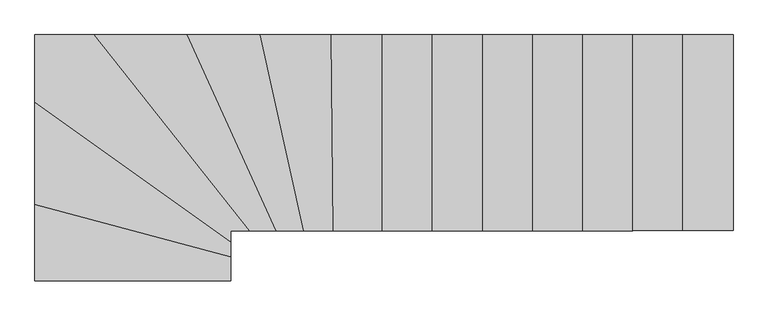
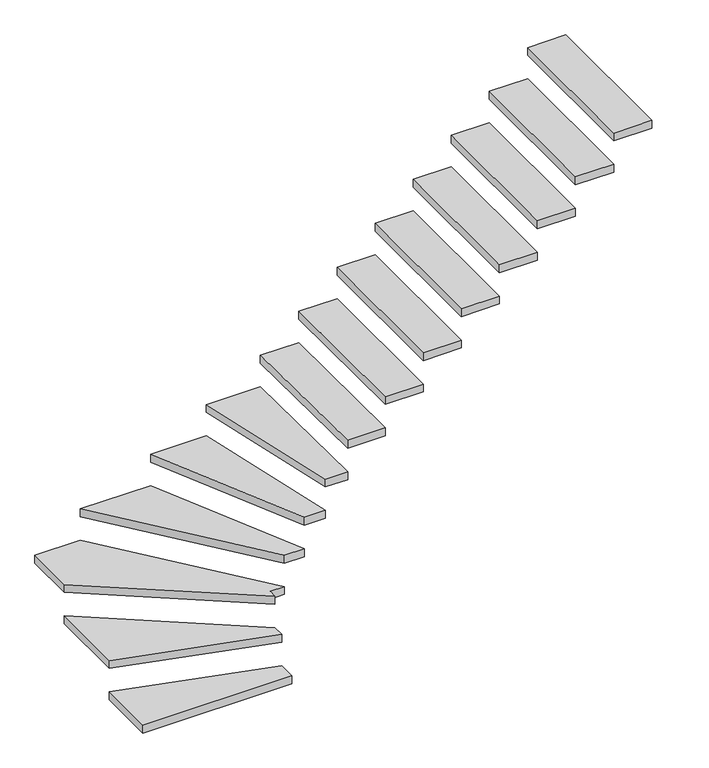
"""IFC4 building model written with IfcOpenShell, lengths in millimetres: stair geometry,   149542 :   149542."""

import ifcopenshell
import ifcopenshell.guid

model = None  # the IFC model being written
_history = None  # IfcOwnerHistory: only IFC2X3 demands one
_inside = {}  # id of a spatial element -> (the spatial element, [elements in it])
_under = {}  # id of a project, library or spatial element -> (it, [spatial elements below it])
_declared = {}  # id of a project -> (the project, [libraries it declares])
_typed = {}  # id of a type object -> (the type object, [elements of that type])
_made_of = {}  # id of a material, layer set ... -> (it, [elements and type objects made of it])


def new_model(schema):
    """Start an empty IFC model of exactly this schema.

    Asked for "IFC4X3", IfcOpenShell would pick the latest addendum, in which some entities
    have other attributes; the version numbers below select the first issue.
    IFC2X3 requires an IfcOwnerHistory on every rooted entity: one is made here for all.
    """
    global model, _history
    if schema == "IFC4X3":
        model = ifcopenshell.file(schema_version=(4, 3, 0, 0))
    else:
        model = ifcopenshell.file(schema=schema)
    _inside.clear()
    _under.clear()
    _declared.clear()
    _typed.clear()
    _made_of.clear()
    _history = None
    if model.schema == "IFC2X3":
        org = make("IfcOrganization", Name="unknown")
        user = make(
            "IfcPersonAndOrganization",
            ThePerson=make("IfcPerson", FamilyName="unknown"),
            TheOrganization=org,
        )
        app = make(
            "IfcApplication",
            ApplicationDeveloper=org,
            Version="unknown",
            ApplicationFullName="unknown",
            ApplicationIdentifier="unknown",
        )
        _history = make(
            "IfcOwnerHistory",
            OwningUser=user,
            OwningApplication=app,
            ChangeAction="ADDED",
            CreationDate=0,
        )
    return model


def make(cls, **values):
    """One entity of the class cls with the attributes given. An attribute that is None is left unset."""
    return model.create_entity(
        cls, **{name: value for name, value in values.items() if value is not None}
    )


def rooted(cls, **values):
    """An entity with a GlobalId (a new one), such as an element, a storey or a relation."""
    return make(cls, GlobalId=ifcopenshell.guid.new(), OwnerHistory=_history, **values)


def si_unit(unit_type, name, prefix=None):
    """IfcSIUnit, for example si_unit("LENGTHUNIT", "METRE", prefix="MILLI")."""
    return make("IfcSIUnit", UnitType=unit_type, Prefix=prefix, Name=name)


def assignment(units):
    """IfcUnitAssignment: the units of a project."""
    return None if units is None else make("IfcUnitAssignment", Units=units)


def point(xyz):
    """IfcCartesianPoint."""
    return None if xyz is None else make("IfcCartesianPoint", Coordinates=xyz)


def direction(xyz):
    """IfcDirection."""
    return None if xyz is None else make("IfcDirection", DirectionRatios=xyz)


def frame(location, z_axis=None, x_axis=None):
    """IfcAxis2Placement3D, a coordinate frame: its origin and axes. An axis left out is left unset."""
    return make(
        "IfcAxis2Placement3D",
        Location=point(location),
        Axis=direction(z_axis),
        RefDirection=direction(x_axis),
    )


def origin():
    """The frame at (0, 0, 0) with its axes left unset."""
    return frame((0.0, 0.0, 0.0))


def place(relative_to, where):
    """IfcLocalPlacement: puts the frame where relative to a parent placement (None: the world)."""
    return make(
        "IfcLocalPlacement", PlacementRelTo=relative_to, RelativePlacement=where
    )


def context(
    kind, dimensions, precision=None, world=None, true_north=None, identifier=None
):
    """IfcGeometricRepresentationContext, for example the 3D "Model" context."""
    return make(
        "IfcGeometricRepresentationContext",
        ContextIdentifier=identifier,
        ContextType=kind,
        CoordinateSpaceDimension=dimensions,
        Precision=precision,
        WorldCoordinateSystem=world,
        TrueNorth=true_north,
    )


def project(units=None, contexts=None):
    """IfcProject with its units and contexts."""
    return rooted(
        "IfcProject",
        Name="project",
        RepresentationContexts=contexts,
        UnitsInContext=assignment(units),
    )


def spatial(cls, under=None, at=None, **own):
    """A site, building, storey or space (cls), placed at a placement, below another one or the project."""
    s = rooted(cls, ObjectPlacement=at, **own)
    if under is not None:
        _under.setdefault(under.id(), (under, []))[1].append(s)
    return s


def polyline(points):
    """IfcPolyline through the points."""
    return make("IfcPolyline", Points=[point(p) for p in points])


def outline(outer, holes=None, kind="AREA"):
    """IfcArbitraryClosedProfileDef: a profile drawn as a closed curve; with holes, ...WithVoids."""
    if holes is None:
        return make("IfcArbitraryClosedProfileDef", ProfileType=kind, OuterCurve=outer)
    return make(
        "IfcArbitraryProfileDefWithVoids",
        ProfileType=kind,
        OuterCurve=outer,
        InnerCurves=holes,
    )


def extrude(swept, where, along, depth):
    """IfcExtrudedAreaSolid: the profile swept, set in the frame where, extruded along a direction by depth."""
    return make(
        "IfcExtrudedAreaSolid",
        SweptArea=swept,
        Position=where,
        ExtrudedDirection=direction(along),
        Depth=depth,
    )


def shape(context_of_items, identifier, shape_type, items):
    """IfcShapeRepresentation: the items that make up one representation, for example the "Body"."""
    return make(
        "IfcShapeRepresentation",
        ContextOfItems=context_of_items,
        RepresentationIdentifier=identifier,
        RepresentationType=shape_type,
        Items=items,
    )


def source(mapping_origin, context_of_items, identifier, shape_type, items):
    """IfcRepresentationMap: a shape defined once, which mapped items show again and again."""
    return make(
        "IfcRepresentationMap",
        MappingOrigin=mapping_origin,
        MappedRepresentation=shape(context_of_items, identifier, shape_type, items),
    )


def transform(
    local_origin,
    x_axis=None,
    y_axis=None,
    z_axis=None,
    scale=None,
    scale2=None,
    scale3=None,
    uniform=True,
):
    """IfcCartesianTransformationOperator3D, or its non-uniform kind. x_axis, y_axis, z_axis: its Axis1, 2, 3."""
    if uniform:
        return make(
            "IfcCartesianTransformationOperator3D",
            Axis1=direction(x_axis),
            Axis2=direction(y_axis),
            LocalOrigin=point(local_origin),
            Scale=scale,
            Axis3=direction(z_axis),
        )
    return make(
        "IfcCartesianTransformationOperator3DnonUniform",
        Axis1=direction(x_axis),
        Axis2=direction(y_axis),
        LocalOrigin=point(local_origin),
        Scale=scale,
        Axis3=direction(z_axis),
        Scale2=scale2,
        Scale3=scale3,
    )


def mapped(mapping_source, mapping_target):
    """IfcMappedItem: shows the shape of a source again, moved by a transform."""
    return make(
        "IfcMappedItem", MappingSource=mapping_source, MappingTarget=mapping_target
    )


def made_of(thing, what):
    """Note that an element or type object is made of a material, layer set ...; save() writes the relation."""
    if what is not None:
        _made_of.setdefault(what.id(), (what, []))[1].append(thing)
    return thing


def element(
    cls,
    number,
    at=None,
    inside=None,
    cuts=None,
    type_object=None,
    material=None,
    context=None,
    identifier="Body",
    shape_type=None,
    held_by="IfcProductDefinitionShape",
    body=None,
    shapes=None,
    **own,
):
    """One element of the class cls, such as IfcWall. Its Tag is "e" and its number.

    at: its placement. inside: the storey or other place that contains it. cuts: it is an
    opening in that element (IfcRelVoidsElement). A single representation is given by context,
    identifier, shape_type and body (its items); several are given by shapes. held_by: the class
    of the entity that holds the representations. save() writes the other relations.
    """
    e = rooted(cls, Tag="e%d" % number, ObjectPlacement=at, **own)
    if body is not None:
        shapes = [shape(context, identifier, shape_type, body)]
    if shapes is not None:
        e.Representation = make(held_by, Representations=shapes)
    if inside is not None:
        _inside.setdefault(inside.id(), (inside, []))[1].append(e)
    if cuts is not None:
        rooted(
            "IfcRelVoidsElement", RelatingBuildingElement=cuts, RelatedOpeningElement=e
        )
    if type_object is not None:
        _typed.setdefault(type_object.id(), (type_object, []))[1].append(e)
    return made_of(e, material)


def aggregate(whole, parts):
    """IfcRelAggregates: a whole, such as a stair, and the parts it consists of."""
    return rooted("IfcRelAggregates", RelatingObject=whole, RelatedObjects=parts)


def save(model, path):
    """Write the relations noted so far, then the file.

    IfcRelAggregates (storeys below a building ...), IfcRelContainedInSpatialStructure (elements
    in a storey), IfcRelDefinesByType, IfcRelAssociatesMaterial and IfcRelDeclares: one each for
    every whole, place, type object, material and project.
    """
    for whole, parts in _under.values():
        aggregate(whole, parts)
    for where, things in _inside.values():
        rooted(
            "IfcRelContainedInSpatialStructure",
            RelatedElements=things,
            RelatingStructure=where,
        )
    for kind, things in _typed.values():
        rooted("IfcRelDefinesByType", RelatedObjects=things, RelatingType=kind)
    for what, things in _made_of.values():
        rooted("IfcRelAssociatesMaterial", RelatedObjects=things, RelatingMaterial=what)
    for by, libraries in _declared.values():
        rooted("IfcRelDeclares", RelatingContext=by, RelatedDefinitions=libraries)
    model.write(path)


def stair_92ba3d55(model_context):
    return source(origin(), model_context, "Body", "SweptSolid", [
        extrude(outline(polyline([(160077.7593015, 32139.1812131), (160077.7593015, 32029.7962965), (159177.7593015, 32029.7962965), (159177.7593015, 32381.5903923), (160077.7593015, 32139.1812131)])), frame((0.0, 0.0, 3480.0), z_axis=(0.0, 0.0, 1.0), x_axis=(1.0, 0.0, 0.0)), (0.0, 0.0, 1.0), 50.0),
        extrude(outline(polyline([(160077.7593015, 32208.6851854), (160077.7593015, 32139.1812131), (159177.7593015, 32381.5903923), (159177.7593015, 32851.1265298), (160077.7593015, 32208.6851854)])), frame((0.0, 0.0, 3680.0), z_axis=(0.0, 0.0, 1.0), x_axis=(1.0, 0.0, 0.0)), (0.0, 0.0, 1.0), 50.0),
        extrude(outline(polyline([(159450.38828, 33159.7962965), (160164.4298971, 32259.7962965), (160077.7593015, 32259.7962965), (160077.7593015, 32208.6851854), (159177.7593015, 32851.1265298), (159177.7593015, 33159.7962965), (159450.38828, 33159.7962965)])), frame((0.0, 0.0, 3880.0), z_axis=(0.0, 0.0, 1.0), x_axis=(1.0, 0.0, 0.0)), (0.0, 0.0, 1.0), 50.0),
        extrude(outline(polyline([(160285.4396784, 32259.7962965), (160164.4298971, 32259.7962965), (159450.38828, 33159.7962965), (159877.5404106, 33159.7962965), (160285.4396784, 32259.7962965)])), frame((0.0, 0.0, 4080.0), z_axis=(0.0, 0.0, 1.0), x_axis=(1.0, 0.0, 0.0)), (0.0, 0.0, 1.0), 50.0),
        extrude(outline(polyline([(160412.2916695, 32259.7962965), (160285.4396784, 32259.7962965), (159877.5404106, 33159.7962965), (160212.4306066, 33159.7962965), (160412.2916695, 32259.7962965)])), frame((0.0, 0.0, 4280.0), z_axis=(0.0, 0.0, 1.0), x_axis=(1.0, 0.0, 0.0)), (0.0, 0.0, 1.0), 50.0),
        extrude(outline(polyline([(160546.5910216, 32259.7962965), (160412.2916695, 32259.7962965), (160212.4306066, 33159.7962965), (160538.1312545, 33159.7962965), (160546.5910216, 32259.7962965)])), frame((0.0, 0.0, 4480.0), z_axis=(0.0, 0.0, 1.0), x_axis=(1.0, 0.0, 0.0)), (0.0, 0.0, 1.0), 50.0),
        extrude(outline(polyline([(160772.3611381, 32259.7962965), (160546.5910216, 32259.7962965), (160538.1312545, 33159.7962965), (160772.3611381, 33159.7962965), (160772.3611381, 32259.7962965)])), frame((0.0, 0.0, 4680.0), z_axis=(0.0, 0.0, 1.0), x_axis=(1.0, 0.0, 0.0)), (0.0, 0.0, 1.0), 50.0),
        extrude(outline(polyline([(161002.3611381, 32259.7962965), (160772.3611381, 32259.7962965), (160772.3611381, 33159.7962965), (161002.3611381, 33159.7962965), (161002.3611381, 32259.7962965)])), frame((0.0, 0.0, 4880.0), z_axis=(0.0, 0.0, 1.0), x_axis=(1.0, 0.0, 0.0)), (0.0, 0.0, 1.0), 50.0),
        extrude(outline(polyline([(161232.3611381, 32259.7962965), (161002.3611381, 32259.7962965), (161002.3611381, 33159.7962965), (161232.3611381, 33159.7962965), (161232.3611381, 32259.7962965)])), frame((0.0, 0.0, 5080.0), z_axis=(0.0, 0.0, 1.0), x_axis=(1.0, 0.0, 0.0)), (0.0, 0.0, 1.0), 50.0),
        extrude(outline(polyline([(161462.3611381, 32259.7962965), (161232.3611381, 32259.7962965), (161232.3611381, 33159.7962965), (161462.3611381, 33159.7962965), (161462.3611381, 32259.7962965)])), frame((0.0, 0.0, 5280.0), z_axis=(0.0, 0.0, 1.0), x_axis=(1.0, 0.0, 0.0)), (0.0, 0.0, 1.0), 50.0),
        extrude(outline(polyline([(161692.3611381, 32259.7962965), (161462.3611381, 32259.7962965), (161462.3611381, 33159.7962965), (161692.3611381, 33159.7962965), (161692.3611381, 32259.7962965)])), frame((0.0, 0.0, 5480.0), z_axis=(0.0, 0.0, 1.0), x_axis=(1.0, 0.0, 0.0)), (0.0, 0.0, 1.0), 50.0),
        extrude(outline(polyline([(161922.3611381, 32259.7962965), (161692.3611381, 32259.7962965), (161692.3611381, 33159.7962965), (161922.3611381, 33159.7962965), (161922.3611381, 32259.7962965)])), frame((0.0, 0.0, 5680.0), z_axis=(0.0, 0.0, 1.0), x_axis=(1.0, 0.0, 0.0)), (0.0, 0.0, 1.0), 50.0),
        extrude(outline(polyline([(162152.3611381, 32259.7962965), (161922.3611381, 32259.7962965), (161922.3611381, 33159.7962965), (162152.3611381, 33159.7962965), (162152.3611381, 32259.7962965)])), frame((0.0, 0.0, 5880.0), z_axis=(0.0, 0.0, 1.0), x_axis=(1.0, 0.0, 0.0)), (0.0, 0.0, 1.0), 50.0),
        extrude(outline(polyline([(162382.3611381, 32259.7962965), (162152.3611381, 32259.7962965), (162152.3611381, 33159.7962965), (162382.3611381, 33159.7962965), (162382.3611381, 32259.7962965)])), frame((0.0, 0.0, 6080.0), z_axis=(0.0, 0.0, 1.0), x_axis=(1.0, 0.0, 0.0)), (0.0, 0.0, 1.0), 50.0),
    ])


if __name__ == "__main__":
    model = new_model("IFC4")
    model_context = context("Model", 3, world=origin())
    ifc_project = project(units=[si_unit("LENGTHUNIT", "METRE", prefix="MILLI")], contexts=[model_context])
    site = spatial("IfcSite", under=ifc_project)
    building = spatial("IfcBuilding", under=site)
    placement = place(None, origin())
    stair_shape = stair_92ba3d55(model_context)
    element("IfcStair", 1, ObjectType="  149542 :   149542", at=placement, inside=building, context=model_context, shape_type="MappedRepresentation", body=[
        mapped(stair_shape, transform((0.0, 0.0, 0.0), x_axis=(1.0, 0.0, 0.0), y_axis=(0.0, 1.0, 0.0), z_axis=(0.0, 0.0, 1.0))),
    ])
    save(model, "model.ifc")

# Revit data of these elements
# Type "  149542 :   149542"
#   Abrechnungsart = "St"
#   Allright_Bauteil_ID = "0131Tre0659044515"
#   Material = "Stahlbeton"
#   Objektname = "Treppe"
#   NameOverride = " "
#   ThermalTransmittance = 0.0000 BTU/(h·ft²·°F)
#   NosingLength = 0.000 m
#   NumberOfRiser = 14
#   NumberOfTreads = 14
#   RiserHeight = 2.000 m
#   TreadLength = 2.300 m
#   IsExternal = no
#   FireExit = no
#   HandicapAccessible = no
#   HasNonSkidSurface = no
# Element 1 (IfcStair, "  149542 :   149542")
#   Materials on its faces: "weiss"
# Materials
#   "weiss": class "Unassigned", colour RGB 255 255 255, transparency 0
